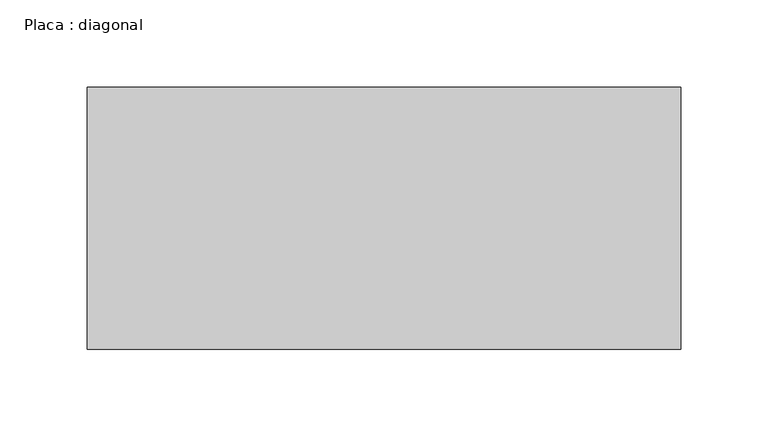
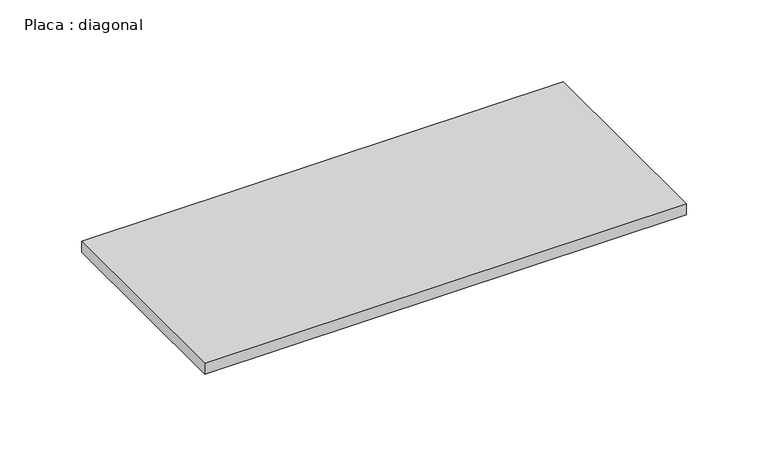
"""IFC4 building model written with IfcOpenShell, lengths in millimetres: beam geometry, Placa : diagonal."""

from ifc_helpers import new_model, si_unit, frame, origin, place, context, project, spatial, polyline, outline, extrude, source, transform, mapped, element, save


def placa_diagonal_9b2e6b67(model_context):
    return source(origin(), model_context, "Body", "SweptSolid", [
        extrude(outline(polyline([(169.9719577, 75.0), (169.9719577, -75.0), (-169.573923, -75.0), (-169.573923, 75.0), (169.9719577, 75.0)])), frame((0.0, 0.0, -4.0), z_axis=(0.0, 0.0, 1.0), x_axis=(1.0, 0.0, 0.0)), (0.0, 0.0, 1.0), 8.0),
    ])


if __name__ == "__main__":
    model = new_model("IFC4")
    model_context = context("Model", 3, world=origin())
    ifc_project = project(units=[si_unit("LENGTHUNIT", "METRE", prefix="MILLI")], contexts=[model_context])
    site = spatial("IfcSite", under=ifc_project)
    building = spatial("IfcBuilding", under=site)
    placement = place(None, origin())
    placa_diagonal_shape = placa_diagonal_9b2e6b67(model_context)
    element("IfcBeam", 1, ObjectType="Placa : diagonal", at=placement, inside=building, context=model_context, shape_type="MappedRepresentation", body=[
        mapped(placa_diagonal_shape, transform((0.0, 0.0, 0.0), x_axis=(1.0, 0.0, 0.0), y_axis=(0.0, 1.0, 0.0), z_axis=(0.0, 0.0, 1.0))),
    ])
    save(model, "model.ifc")

# Revit data of these elements
# Type "Placa : diagonal"
#   W = 0
#   Length [instance default] = 1.50 m
#   b = 0.15 m
#   d = 0.008 m
#   A = 0 m²
#   Structural Material [instance default] = Aço, 45-345
# Element 1 (IfcBeam, "Placa : diagonal")
#   Materials on its faces: "Aço, 45-345"
# Materials
#   "Aço, 45-345": class "Metal", colour RGB 247 247 247, transparency 0, Description = "Aço 345 MPa", Cost = 0
